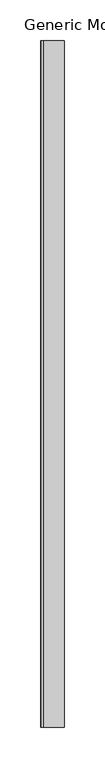
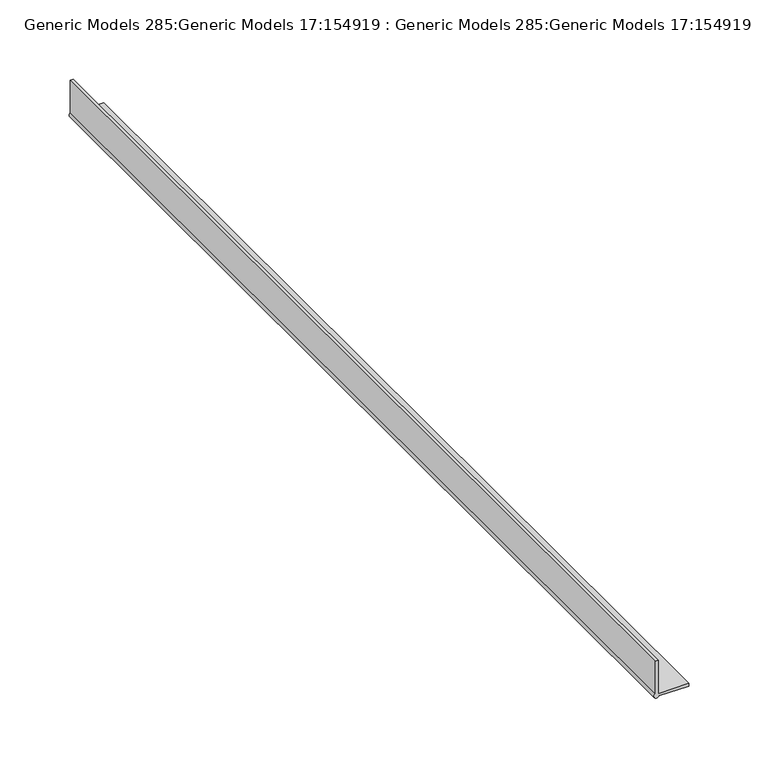
"""IFC4 building model written with IfcOpenShell, lengths in millimetres: proxy geometry, Generic Models 285:Generic Models 17:154919 : Generic Models 285:Generic Models 17:154919."""

from ifc_helpers import new_model, si_unit, point, frame, frame_2d, origin, place, context, project, spatial, polyline, circle_curve, trimmed, segment, composite_curve, outline, extrude, source, transform, mapped, element, save


def generic_models_285_generic_models_17_154919_generic_models_f38c2802(model_context):
    return source(origin(), model_context, "Body", "SweptSolid", [
        extrude(outline(composite_curve([segment(trimmed(circle_curve(frame_2d((5837.3770275, 1421.4076917)), 2.1956516), [point((5839.2075447, 1420.1952178))], [point((5836.3800253, 1423.3639312))], False, "CARTESIAN"), True, "CONTINUOUS"), segment(polyline([(5836.3800253, 1423.3639312), (5836.3800253, 1448.2058187), (5838.6259659, 1448.2058187), (5838.6259659, 1422.6399618), (5868.1300253, 1422.6399618), (5868.1300253, 1420.1952178), (5839.2075447, 1420.1952178)]), True, "CONTINUOUS")], self_intersect=False)), frame((0.0, 4097.6531132, 0.0), z_axis=(0.0, 1.0, 0.0), x_axis=(0.0, 0.0, 1.0)), (0.0, 0.0, 1.0), 846.0415953),
    ])


if __name__ == "__main__":
    model = new_model("IFC4")
    model_context = context("Model", 3, world=origin())
    ifc_project = project(units=[si_unit("LENGTHUNIT", "METRE", prefix="MILLI")], contexts=[model_context])
    site = spatial("IfcSite", under=ifc_project)
    building = spatial("IfcBuilding", under=site)
    placement = place(None, origin())
    generic_models_285_generic_models_17_154919_generic_models_shape = generic_models_285_generic_models_17_154919_generic_models_f38c2802(model_context)
    element("IfcBuildingElementProxy", 1, Name="Generic Models 285:Generic Models 17:154919 : Generic Models 285:Generic Models 17:154919", ObjectType="Generic Models 285:Generic Models 17:154919 : Generic Models 285:Generic Models 17:154919", at=placement, inside=building, context=model_context, shape_type="MappedRepresentation", body=[
        mapped(generic_models_285_generic_models_17_154919_generic_models_shape, transform((0.0, 0.0, 0.0), x_axis=(1.0, 0.0, 0.0), y_axis=(0.0, 1.0, 0.0), z_axis=(0.0, 0.0, 1.0))),
    ])
    save(model, "model.ifc")

# Revit data of these elements
# Type "Generic Models 285:Generic Models 17:154919 : Generic Models 285:Generic Models 17:154919"
#   NameOverride = "Generic Models 285:Generic Models 17:154919"
#   ObjectTypeOverride = "Generic Models 285:Generic Models 17"
#   Reference = "Generic Models 17"
#   Category = "Generic Models"
#   Tag = "154919"
# Element 1 (IfcBuildingElementProxy, "Generic Models 285:Generic Models 17:154919 : Generic Models 285:Generic Models 17:154919")
#   Materials on its faces: "_DRYWALL CORNER BEAD 25414"
# Materials
#   "_DRYWALL CORNER BEAD 25414": class "Unassigned", colour RGB 253 192 103, transparency 0
